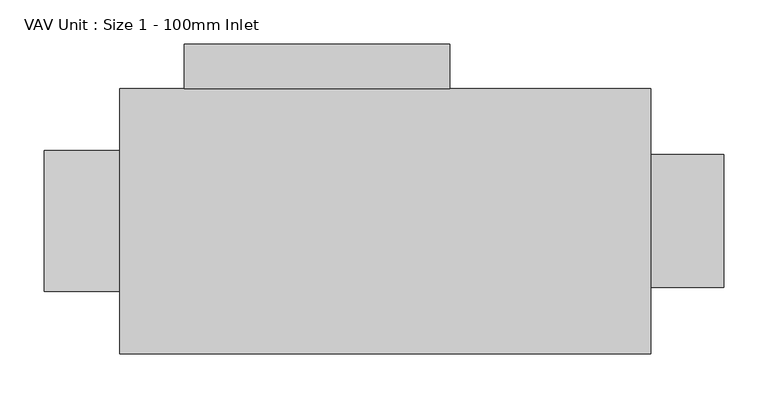
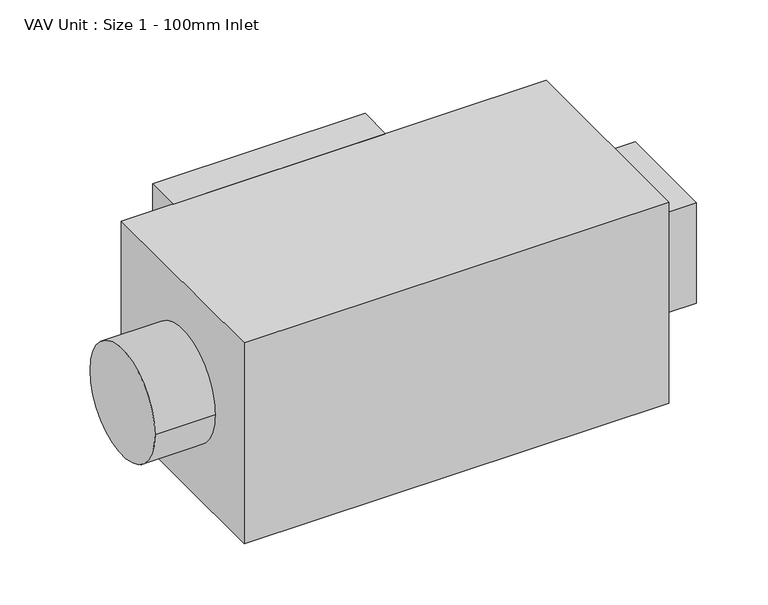
"""IFC4 building model written with IfcOpenShell, lengths in millimetres: proxy geometry, VAV Unit : Size 1 - 100mm Inlet."""

from ifc_helpers import new_model, si_unit, point, frame, origin, origin_2d, place, context, project, spatial, polyline, circle_curve, trimmed, segment, composite_curve, outline, extrude, source, transform, mapped, element, save


def vav_unit_size_1_100mm_inlet_d2cd518a(model_context):
    return source(origin(), model_context, "Body", "SweptSolid", [
        extrude(outline(polyline([(382.4821717, 75.0), (382.4821717, -75.0), (300.0, -75.0), (300.0, 75.0), (382.4821717, 75.0)])), frame((0.0, 0.0, -75.0), z_axis=(0.0, 0.0, 1.0), x_axis=(1.0, 0.0, 0.0)), (0.0, 0.0, 1.0), 150.0),
        extrude(outline(polyline([(73.0, 150.0), (-227.0, 150.0), (-227.0, 200.0), (73.0, 200.0), (73.0, 150.0)])), frame((0.0, 0.0, -150.0), z_axis=(0.0, 0.0, 1.0), x_axis=(1.0, 0.0, 0.0)), (0.0, 0.0, 1.0), 300.0),
        extrude(outline(composite_curve([segment(trimmed(circle_curve(origin_2d(), 79.5), [point((-79.5, 0.0))], [point((79.5, 0.0))], False, "CARTESIAN"), True, "CONTINUOUS"), segment(trimmed(circle_curve(origin_2d(), 79.5), [point((79.5, 0.0))], [point((-79.5, 0.0))], False, "CARTESIAN"), True, "CONTINUOUS")], self_intersect=False)), frame((-385.0, 0.0, 0.0), z_axis=(1.0, 0.0, 0.0), x_axis=(0.0, 1.0, 0.0)), (0.0, 0.0, 1.0), 85.0),
        extrude(outline(polyline([(300.0, 150.0), (300.0, -150.0), (-300.0, -150.0), (-300.0, 150.0), (300.0, 150.0)])), frame((0.0, 0.0, -150.0), z_axis=(0.0, 0.0, 1.0), x_axis=(1.0, 0.0, 0.0)), (0.0, 0.0, 1.0), 300.0),
    ])


if __name__ == "__main__":
    model = new_model("IFC4")
    model_context = context("Model", 3, world=origin())
    ifc_project = project(units=[si_unit("LENGTHUNIT", "METRE", prefix="MILLI")], contexts=[model_context])
    site = spatial("IfcSite", under=ifc_project)
    building = spatial("IfcBuilding", under=site)
    placement = place(None, origin())
    vav_unit_size_1_100mm_inlet_shape = vav_unit_size_1_100mm_inlet_d2cd518a(model_context)
    element("IfcBuildingElementProxy", 1, Name="VAV Unit : Size 1 - 100mm Inlet", ObjectType="VAV Unit : Size 1 - 100mm Inlet", at=placement, inside=building, context=model_context, shape_type="MappedRepresentation", body=[
        mapped(vav_unit_size_1_100mm_inlet_shape, transform((0.0, 0.0, 0.0), x_axis=(1.0, 0.0, 0.0), y_axis=(0.0, 1.0, 0.0), z_axis=(0.0, 0.0, 1.0))),
    ])
    save(model, "model.ifc")

# Revit data of these elements
# Type "VAV Unit : Size 1 - 100mm Inlet"
#   Type Mark = "VAV Unit"
#   COBie.Type.CreatedBy = "info@mma.ie"
#   COBie.Type.CreatedOn = "2017-07-21T10:57:54"
#   COBie.Type.Name = "VAV Unit"
#   COBie.Type.Category = "23-33 41 17 13 : Variable Air Volume Terminal Units"
#   COBie.Type.Description = "VAV Unit_Size 1 - 100mm Inlet"
#   COBie.Type.AssetType = "Fixed"
#   COBie.Type.Manufacturer = ""
#   COBie.Type.ModelNumber = ""
#   COBie.Type.ModelReference = ""
#   Classification.OmniClass.23.Number = "23-33 41 17 13"
#   Classification.OmniClass.23.Description = "Variable Air Volume Terminal Units"
#   Keynote = "23 36 16.A"
#   COBie.Type.ReplacementCost = 0
#   Width2 = 150 mm
#   Voltage = 230 V
#   UnitWidth = 600 mm
#   UnitHeight = 300 mm
#   UnitDepth = 300 mm
#   Unit Weight = 300 mm
#   Unit Lenght = 600 mm
#   Unit Height = 300 mm
#   SupplyConnectorWidth = 150 mm
#   SupplyConnectorVerticalOffset = 54 mm
#   SupplyConnectorLength = 15 mm
#   SupplyConnectorHorizontalOffset = 90 mm
#   SupplyConnectorDepth = 150 mm
#   SupplyAirConnectorCenterOffset = 165 mm
#   Static Pressure [instance default] = 0.0401865 in-wg
#   PrimaryToSupplyRatio [instance default] = 0.2
#   PrimaryAirOffset = 150 mm
#   PrimaryAirFlow [instance default] = 100.011 CFM
#   PrimaryAirConnectorVerticalOffset = 150 mm
#   PrimaryAirConnectorRadius = 79.5 mm
#   PrimaryAirConnectorLength = 85 mm
#   PrimaryAirConnectorDiameter = 159 mm
#   PrimaryAirConnectorCenterOffset = 150 mm
#   InducedAirInletWidth = 400 mm
#   InducedAirInletDepth = 350 mm
#   InducedAirConnectorHorizontalOffset = 25 mm
#   InducedAirConnectorCenterOffset = 225 mm
#   Height2 = 150 mm
#   ElectricalConnectionBoxWidth = 300 mm
#   ElectricalConnectionBoxOffset = 73 mm
#   ElectricalConnectionBoxHeight = 50 mm
#   ElectricalConnectionBoxDepth = 300 mm
#   Apparent Load = 181 VA
#   Air Flow [instance default] = 500.056 CFM
#   COBie.Type = yes
#   SupplyAirConnectorIndex = 2
#   PrimaryAirConnectorIndex = 1
#   Number of Poles = 1
#   InducedAirConnectorIndex = 3
#   VAV Material = none
#   Load Classification = Cooling
#   Default Elevation = 0
#   Assembly Code = ""
# Element 1 (IfcBuildingElementProxy, "VAV Unit : Size 1 - 100mm Inlet")
#   Static Pressure = 0.1 in-wg
#   PrimaryAirFlow = 298.762 CFM
#   Air Flow = 1493.81 CFM
